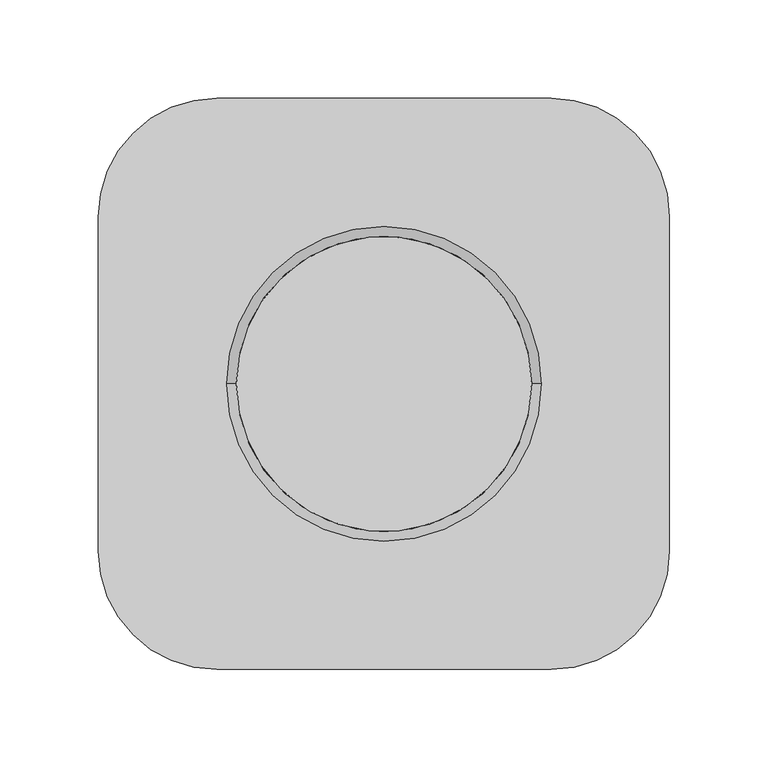
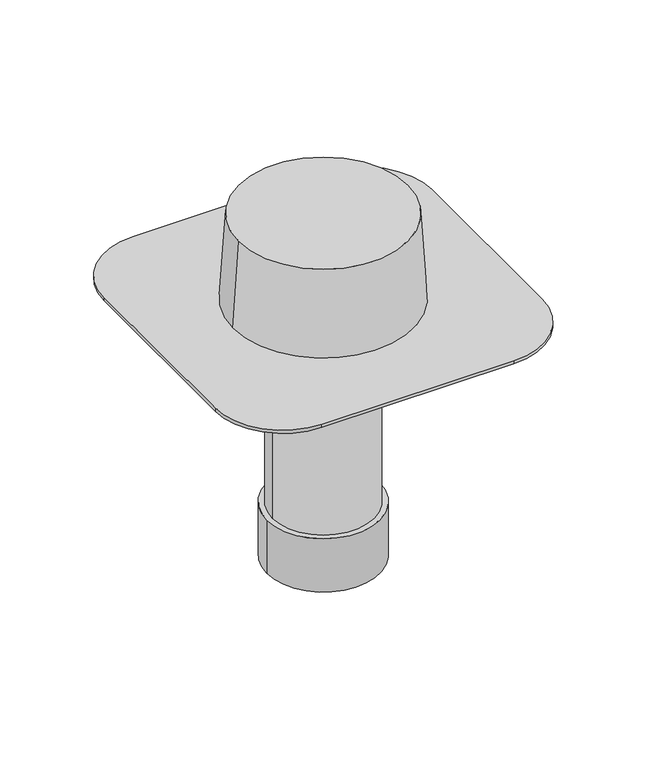
"""IFC4 building model written with IfcOpenShell, lengths in millimetres: proxy geometry, TN_Воронка ТехноНИКОЛЬ ремонтная : Воронка ТехноНИКОЛЬ ремонтная c уплотнителем, 90Х240."""

from ifc_helpers import new_model, si_unit, point, frame, origin, origin_2d, place, context, project, spatial, polyline, circle_curve, trimmed, segment, composite_curve, outline, extrude, source, transform, mapped, element, save
from ifc_brep_helpers import plane_surface, cylinder_surface, revolved_surface, advanced_brep


def specialty_equipment_e63e5d4e(model_context):
    return source(origin(), model_context, "Body", "SolidModel", [
        extrude(outline(composite_curve([segment(trimmed(circle_curve(origin_2d(), 50.0), [point((50.0, 0.0))], [point((-50.0, 0.0))], False, "CARTESIAN"), True, "CONTINUOUS"), segment(trimmed(circle_curve(origin_2d(), 50.0), [point((-50.0, 0.0))], [point((50.0, 0.0))], False, "CARTESIAN"), True, "CONTINUOUS")], self_intersect=False), holes=[composite_curve([segment(trimmed(circle_curve(origin_2d(), 45.0), [point((45.0, 0.0))], [point((-45.0, 0.0))], True, "CARTESIAN"), True, "CONTINUOUS"), segment(trimmed(circle_curve(origin_2d(), 45.0), [point((-45.0, 0.0))], [point((45.0, 0.0))], True, "CARTESIAN"), True, "CONTINUOUS")], self_intersect=False)]), frame((0.0, 0.0, -240.0), z_axis=(0.0, 0.0, 1.0), x_axis=(1.0, 0.0, 0.0)), (0.0, 0.0, 1.0), 50.0),
        advanced_brep(
        [(0.0, 0.0, -240.0), (-45.0, 0.0, -240.0), (45.0, 0.0, -240.0), (-45.0, 0.0, -3.0), (45.0, 0.0, -3.0), (85.0, 145.0, -3.0), (145.0, 85.0, -3.0), (145.0, -85.0, -3.0), (85.0, -145.0, -3.0), (-85.0, -145.0, -3.0), (-145.0, -85.0, -3.0), (-145.0, 85.0, -3.0), (-85.0, 145.0, -3.0), (85.0, 145.0, 0.0), (-85.0, 145.0, 0.0), (-145.0, 85.0, 0.0), (-145.0, -85.0, 0.0), (-85.0, -145.0, 0.0), (85.0, -145.0, 0.0), (145.0, -85.0, 0.0), (145.0, 85.0, 0.0)],
        [
            (0, 1),
            (1, 2, circle_curve(frame((0.0, 0.0, -240.0), z_axis=(0.0, 0.0, -1.0), x_axis=(-1.0, 0.0, 0.0)), 45.0)),
            (2, 0),
            (2, 1, circle_curve(frame((0.0, 0.0, -240.0), z_axis=(0.0, 0.0, -1.0), x_axis=(-1.0, 0.0, 0.0)), 45.0)),
            (1, 3),
            (3, 4, circle_curve(frame((0.0, 0.0, -3.0), z_axis=(0.0, 0.0, -1.0), x_axis=(-1.0, 0.0, 0.0)), 45.0)),
            (4, 2),
            (4, 3, circle_curve(frame((0.0, 0.0, -3.0), z_axis=(0.0, 0.0, -1.0), x_axis=(-1.0, 0.0, 0.0)), 45.0)),
            (5, 6, circle_curve(frame((85.0, 85.0, -3.0), z_axis=(0.0, 0.0, -1.0), x_axis=(1.0, 0.0, 0.0)), 60.0)),
            (6, 7),
            (7, 8, circle_curve(frame((85.0, -85.0, -3.0), z_axis=(0.0, 0.0, -1.0), x_axis=(1.0, 0.0, 0.0)), 60.0)),
            (8, 9),
            (9, 10, circle_curve(frame((-85.0, -85.0, -3.0), z_axis=(0.0, 0.0, -1.0), x_axis=(1.0, 0.0, 0.0)), 60.0)),
            (10, 11),
            (11, 12, circle_curve(frame((-85.0, 85.0, -3.0), z_axis=(0.0, 0.0, -1.0), x_axis=(1.0, 0.0, 0.0)), 60.0)),
            (12, 5),
            (13, 14),
            (14, 15, circle_curve(frame((-85.0, 85.0, 0.0), z_axis=(0.0, 0.0, 1.0), x_axis=(1.0, 0.0, 0.0)), 60.0)),
            (15, 16),
            (16, 17, circle_curve(frame((-85.0, -85.0, 0.0), z_axis=(0.0, 0.0, 1.0), x_axis=(1.0, 0.0, 0.0)), 60.0)),
            (17, 18),
            (18, 19, circle_curve(frame((85.0, -85.0, 0.0), z_axis=(0.0, 0.0, 1.0), x_axis=(1.0, 0.0, 0.0)), 60.0)),
            (19, 20),
            (20, 13, circle_curve(frame((85.0, 85.0, 0.0), z_axis=(0.0, 0.0, 1.0), x_axis=(1.0, 0.0, 0.0)), 60.0)),
            (12, 14),
            (13, 5),
            (10, 16),
            (15, 11),
            (8, 18),
            (17, 9),
            (6, 20),
            (19, 7),
        ],
        [
            plane_surface(frame((0.0, 0.0, -240.0), z_axis=(0.0, 0.0, -1.0), x_axis=(-1.0, 0.0, 0.0))),
            cylinder_surface(frame((0.0, 0.0, 0.0), z_axis=(0.0, 0.0, -1.0), x_axis=(-1.0, 0.0, 0.0)), 45.0),
            plane_surface(frame((-350.0, 145.0, -3.0), z_axis=(0.0, 0.0, -1.0), x_axis=(1.0, 0.0, 0.0))),
            plane_surface(frame((-350.0, 145.0, 0.0), z_axis=(0.0, 0.0, 1.0), x_axis=(-1.0, 0.0, 0.0))),
            plane_surface(frame((85.0, 145.0, 0.0), z_axis=(0.0, 1.0, 0.0), x_axis=(0.0, 0.0, -1.0))),
            plane_surface(frame((-145.0, 85.0, 0.0), z_axis=(-1.0, 0.0, 0.0), x_axis=(0.0, 0.0, -1.0))),
            plane_surface(frame((-85.0, -145.0, 0.0), z_axis=(0.0, -1.0, 0.0), x_axis=(0.0, 0.0, -1.0))),
            plane_surface(frame((145.0, -85.0, 0.0), z_axis=(1.0, 0.0, 0.0), x_axis=(0.0, 0.0, -1.0))),
            cylinder_surface(frame((-85.0, 85.0, -3.0), z_axis=(0.0, 0.0, 1.0), x_axis=(1.0, 0.0, 0.0)), 60.0),
            cylinder_surface(frame((-85.0, -85.0, -3.0), z_axis=(0.0, 0.0, 1.0), x_axis=(1.0, 0.0, 0.0)), 60.0),
            cylinder_surface(frame((85.0, -85.0, -3.0), z_axis=(0.0, 0.0, 1.0), x_axis=(1.0, 0.0, 0.0)), 60.0),
            cylinder_surface(frame((85.0, 85.0, -3.0), z_axis=(0.0, 0.0, 1.0), x_axis=(1.0, 0.0, 0.0)), 60.0),
        ],
        [
            (0, [[1, 2, 3]]),
            (0, [[-1, -3, 4]]),
            (1, [[-2, 5, 6, 7]]),
            (1, [[-4, -7, 8, -5]]),
            (2, [[9, 10, 11, 12, 13, 14, 15, 16], [-6, -8]]),
            (3, [[17, 18, 19, 20, 21, 22, 23, 24]]),
            (4, [[-16, 25, -17, 26]]),
            (5, [[-14, 27, -19, 28]]),
            (6, [[-12, 29, -21, 30]]),
            (7, [[-10, 31, -23, 32]]),
            (8, [[-15, -28, -18, -25]]),
            (9, [[-13, -30, -20, -27]]),
            (10, [[-11, -32, -22, -29]]),
            (11, [[-9, -26, -24, -31]]),
        ],
    ),
        advanced_brep(
        [(-75.0, 0.0, 80.0), (75.0, 0.0, 80.0), (-80.0, 0.0, 0.0), (80.0, 0.0, 0.0)],
        [
            (0, 1, circle_curve(frame((0.0, 0.0, 80.0), z_axis=(0.0, 0.0, 1.0), x_axis=(-1.0, 0.0, 0.0)), 75.0)),
            (1, 0, circle_curve(frame((0.0, 0.0, 80.0), z_axis=(0.0, 0.0, 1.0), x_axis=(1.0, 0.0, 0.0)), 75.0)),
            (2, 3, circle_curve(frame((0.0, 0.0, 0.0), z_axis=(0.0, 0.0, -1.0), x_axis=(1.0, 0.0, 0.0)), 80.0)),
            (3, 2, circle_curve(frame((0.0, 0.0, 0.0), z_axis=(0.0, 0.0, -1.0), x_axis=(-1.0, 0.0, 0.0)), 80.0)),
            (3, 1),
            (0, 2),
        ],
        [
            plane_surface(frame((0.0, 0.0, 80.0), z_axis=(0.0, 0.0, 1.0), x_axis=(0.0, -1.0, 0.0))),
            plane_surface(frame((0.0, 0.0, 0.0), z_axis=(0.0, 0.0, -1.0), x_axis=(0.0, -1.0, 0.0))),
            revolved_surface(polyline([(-75.0, 0.0, 80.0), (-80.0, 0.0, 0.0)]), (0.0, 0.0, 1280.0), (0.0, 0.0, -1.0)),
            revolved_surface(polyline([(75.0, 0.0, 80.0), (80.0, 0.0, 0.0)]), (0.0, 0.0, 1280.0), (0.0, 0.0, -1.0)),
        ],
        [
            (0, [[1, 2]]),
            (1, [[3, 4]]),
            (2, [[-4, 5, -1, 6]]),
            (3, [[-3, -6, -2, -5]]),
        ],
    ),
    ])


if __name__ == "__main__":
    model = new_model("IFC4")
    model_context = context("Model", 3, world=origin())
    ifc_project = project(units=[si_unit("LENGTHUNIT", "METRE", prefix="MILLI")], contexts=[model_context])
    site = spatial("IfcSite", under=ifc_project)
    building = spatial("IfcBuilding", under=site)
    placement = place(None, origin())
    specialty_equipment_shape = specialty_equipment_e63e5d4e(model_context)
    element("IfcBuildingElementProxy", 1, Name="TN_Воронка ТехноНИКОЛЬ ремонтная : Воронка ТехноНИКОЛЬ ремонтная c уплотнителем, 90Х240", ObjectType="TN_Воронка ТехноНИКОЛЬ ремонтная : Воронка ТехноНИКОЛЬ ремонтная c уплотнителем, 90Х240", at=placement, inside=building, context=model_context, shape_type="MappedRepresentation", body=[
        mapped(specialty_equipment_shape, transform((0.0, 0.0, 0.0), x_axis=(1.0, 0.0, 0.0), y_axis=(0.0, 1.0, 0.0), z_axis=(0.0, 0.0, 1.0))),
    ])
    save(model, "model.ifc")

# Revit data of these elements
# Type "TN_Воронка ТехноНИКОЛЬ ремонтная : Воронка ТехноНИКОЛЬ ремонтная c уплотнителем, 90Х240"
#   ADSK_Группирование = "Комплектующие и воронки"
#   Description = "Ремонтная воронка ТехноНИКОЛЬ применяется для восстановления внутреннего водостока с плоских кровель, имеющих системы водослива со стальными, чугунными Ø100мм или пластмассовыми трубами Ø110мм. Воронки могут устанавливаться в кровлю безогневым способом на мастику герметизирующую № 71. Воронка ТехноНИКОЛЬ ремонтная 90х240 используются при ремонте зданий и сооружений с плоскими кровлями. Применяются в кровлях из битумных и битумно-полимерных рулонных и мастичных материалов с внутренним водостоком. Пропускная способность, 7,6 л/сек."
#   Manufacturer = "ТехноНИКОЛЬ"
#   URL = "https://shop.tn.ru/voronka-tehnonikol-remontnaja-c-uplotnitelem-90h240-mm"
#   ADSK_Примечание = ""
#   ADSK_Обозначение = "ТехноНИКОЛЬ"
#   ADSK_Наименование = "Воронка ТехноНИКОЛЬ ремонтная c уплотнителем, 90Х240"
#   ADSK_Марка = ""
#   ADSK_Код изделия = "460064"
#   ADSK_Завод-изготовитель = "ТехноНИКОЛЬ"
#   ADSK_Единица измерения = "шт."
#   ADSK_Группирование = "Комплектующие и воронки"
#   ADSK_URL страницы изделия = "https://shop.tn.ru/voronka-tehnonikol-remontnaja-c-uplotnitelem-90h240-mm"
#   ADSK_URL документации изделия = "https://nav.tn.ru/upload/iblock/5b0/Tekhlist-7.22_Voronka_remontnaya_rus.pdf"
#   Пропускная способность = 7.6 L/s
#   Длина расчетная [instance default] = 240 mm
#   Длина отвода [instance default] = 240 mm
#   Диаметр = 90 mm
#   ADSK_Масса = 0.6
#   ADSK_Количество = 1
#   Уплотнитель = yes
#   Материал = TN_ПВХ_Черный
#   Default Elevation = 0
# Element 1 (IfcBuildingElementProxy, "TN_Воронка ТехноНИКОЛЬ ремонтная : Воронка ТехноНИКОЛЬ ремонтная c уплотнителем, 90Х240")
#   Materials on its faces: "TN_ПВХ_Черный"
# Materials
#   "TN_ПВХ_Черный": class "Типовые", colour RGB 48 48 48, transparency 0, Cost = 0
